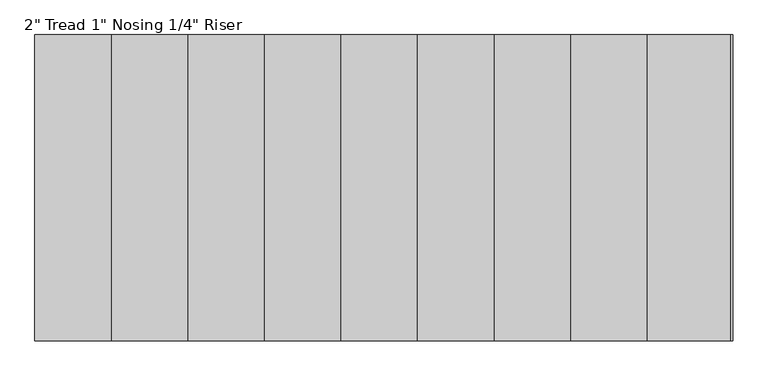
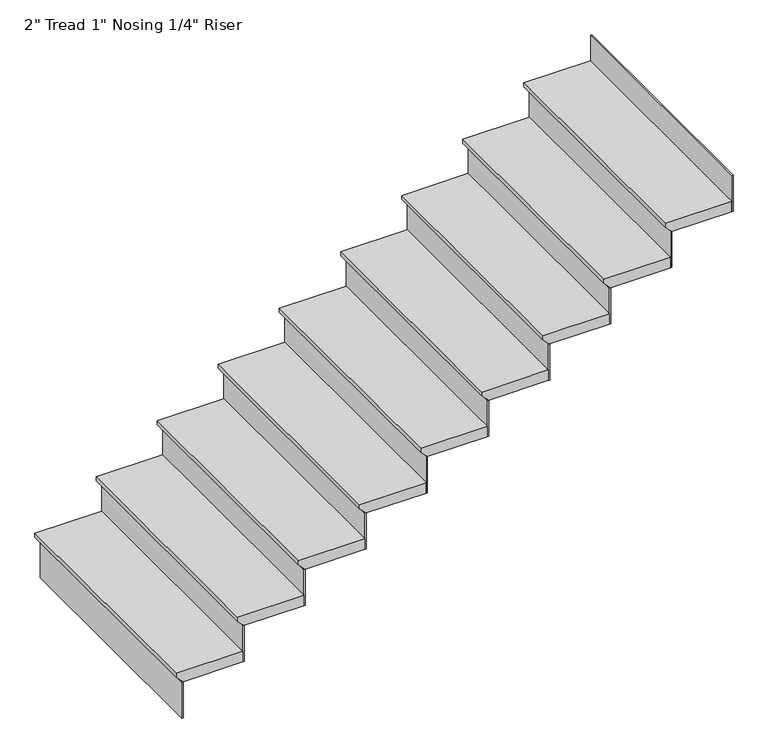
"""IFC4 building model written with IfcOpenShell, lengths in millimetres: stair flight geometry."""

import ifcopenshell
import ifcopenshell.guid

model = None  # the IFC model being written
_history = None  # IfcOwnerHistory: only IFC2X3 demands one
_inside = {}  # id of a spatial element -> (the spatial element, [elements in it])
_under = {}  # id of a project, library or spatial element -> (it, [spatial elements below it])
_declared = {}  # id of a project -> (the project, [libraries it declares])
_typed = {}  # id of a type object -> (the type object, [elements of that type])
_made_of = {}  # id of a material, layer set ... -> (it, [elements and type objects made of it])


def new_model(schema):
    """Start an empty IFC model of exactly this schema.

    Asked for "IFC4X3", IfcOpenShell would pick the latest addendum, in which some entities
    have other attributes; the version numbers below select the first issue.
    IFC2X3 requires an IfcOwnerHistory on every rooted entity: one is made here for all.
    """
    global model, _history
    if schema == "IFC4X3":
        model = ifcopenshell.file(schema_version=(4, 3, 0, 0))
    else:
        model = ifcopenshell.file(schema=schema)
    _inside.clear()
    _under.clear()
    _declared.clear()
    _typed.clear()
    _made_of.clear()
    _history = None
    if model.schema == "IFC2X3":
        org = make("IfcOrganization", Name="unknown")
        user = make(
            "IfcPersonAndOrganization",
            ThePerson=make("IfcPerson", FamilyName="unknown"),
            TheOrganization=org,
        )
        app = make(
            "IfcApplication",
            ApplicationDeveloper=org,
            Version="unknown",
            ApplicationFullName="unknown",
            ApplicationIdentifier="unknown",
        )
        _history = make(
            "IfcOwnerHistory",
            OwningUser=user,
            OwningApplication=app,
            ChangeAction="ADDED",
            CreationDate=0,
        )
    return model


def make(cls, **values):
    """One entity of the class cls with the attributes given. An attribute that is None is left unset."""
    return model.create_entity(
        cls, **{name: value for name, value in values.items() if value is not None}
    )


def rooted(cls, **values):
    """An entity with a GlobalId (a new one), such as an element, a storey or a relation."""
    return make(cls, GlobalId=ifcopenshell.guid.new(), OwnerHistory=_history, **values)


def si_unit(unit_type, name, prefix=None):
    """IfcSIUnit, for example si_unit("LENGTHUNIT", "METRE", prefix="MILLI")."""
    return make("IfcSIUnit", UnitType=unit_type, Prefix=prefix, Name=name)


def assignment(units):
    """IfcUnitAssignment: the units of a project."""
    return None if units is None else make("IfcUnitAssignment", Units=units)


def point(xyz):
    """IfcCartesianPoint."""
    return None if xyz is None else make("IfcCartesianPoint", Coordinates=xyz)


def direction(xyz):
    """IfcDirection."""
    return None if xyz is None else make("IfcDirection", DirectionRatios=xyz)


def frame(location, z_axis=None, x_axis=None):
    """IfcAxis2Placement3D, a coordinate frame: its origin and axes. An axis left out is left unset."""
    return make(
        "IfcAxis2Placement3D",
        Location=point(location),
        Axis=direction(z_axis),
        RefDirection=direction(x_axis),
    )


def origin():
    """The frame at (0, 0, 0) with its axes left unset."""
    return frame((0.0, 0.0, 0.0))


def place(relative_to, where):
    """IfcLocalPlacement: puts the frame where relative to a parent placement (None: the world)."""
    return make(
        "IfcLocalPlacement", PlacementRelTo=relative_to, RelativePlacement=where
    )


def context(
    kind, dimensions, precision=None, world=None, true_north=None, identifier=None
):
    """IfcGeometricRepresentationContext, for example the 3D "Model" context."""
    return make(
        "IfcGeometricRepresentationContext",
        ContextIdentifier=identifier,
        ContextType=kind,
        CoordinateSpaceDimension=dimensions,
        Precision=precision,
        WorldCoordinateSystem=world,
        TrueNorth=true_north,
    )


def project(units=None, contexts=None):
    """IfcProject with its units and contexts."""
    return rooted(
        "IfcProject",
        Name="project",
        RepresentationContexts=contexts,
        UnitsInContext=assignment(units),
    )


def spatial(cls, under=None, at=None, **own):
    """A site, building, storey or space (cls), placed at a placement, below another one or the project."""
    s = rooted(cls, ObjectPlacement=at, **own)
    if under is not None:
        _under.setdefault(under.id(), (under, []))[1].append(s)
    return s


def polyline(points):
    """IfcPolyline through the points."""
    return make("IfcPolyline", Points=[point(p) for p in points])


def outline(outer, holes=None, kind="AREA"):
    """IfcArbitraryClosedProfileDef: a profile drawn as a closed curve; with holes, ...WithVoids."""
    if holes is None:
        return make("IfcArbitraryClosedProfileDef", ProfileType=kind, OuterCurve=outer)
    return make(
        "IfcArbitraryProfileDefWithVoids",
        ProfileType=kind,
        OuterCurve=outer,
        InnerCurves=holes,
    )


def extrude(swept, where, along, depth):
    """IfcExtrudedAreaSolid: the profile swept, set in the frame where, extruded along a direction by depth."""
    return make(
        "IfcExtrudedAreaSolid",
        SweptArea=swept,
        Position=where,
        ExtrudedDirection=direction(along),
        Depth=depth,
    )


def shape(context_of_items, identifier, shape_type, items):
    """IfcShapeRepresentation: the items that make up one representation, for example the "Body"."""
    return make(
        "IfcShapeRepresentation",
        ContextOfItems=context_of_items,
        RepresentationIdentifier=identifier,
        RepresentationType=shape_type,
        Items=items,
    )


def source(mapping_origin, context_of_items, identifier, shape_type, items):
    """IfcRepresentationMap: a shape defined once, which mapped items show again and again."""
    return make(
        "IfcRepresentationMap",
        MappingOrigin=mapping_origin,
        MappedRepresentation=shape(context_of_items, identifier, shape_type, items),
    )


def transform(
    local_origin,
    x_axis=None,
    y_axis=None,
    z_axis=None,
    scale=None,
    scale2=None,
    scale3=None,
    uniform=True,
):
    """IfcCartesianTransformationOperator3D, or its non-uniform kind. x_axis, y_axis, z_axis: its Axis1, 2, 3."""
    if uniform:
        return make(
            "IfcCartesianTransformationOperator3D",
            Axis1=direction(x_axis),
            Axis2=direction(y_axis),
            LocalOrigin=point(local_origin),
            Scale=scale,
            Axis3=direction(z_axis),
        )
    return make(
        "IfcCartesianTransformationOperator3DnonUniform",
        Axis1=direction(x_axis),
        Axis2=direction(y_axis),
        LocalOrigin=point(local_origin),
        Scale=scale,
        Axis3=direction(z_axis),
        Scale2=scale2,
        Scale3=scale3,
    )


def mapped(mapping_source, mapping_target):
    """IfcMappedItem: shows the shape of a source again, moved by a transform."""
    return make(
        "IfcMappedItem", MappingSource=mapping_source, MappingTarget=mapping_target
    )


def made_of(thing, what):
    """Note that an element or type object is made of a material, layer set ...; save() writes the relation."""
    if what is not None:
        _made_of.setdefault(what.id(), (what, []))[1].append(thing)
    return thing


def element(
    cls,
    number,
    at=None,
    inside=None,
    cuts=None,
    type_object=None,
    material=None,
    context=None,
    identifier="Body",
    shape_type=None,
    held_by="IfcProductDefinitionShape",
    body=None,
    shapes=None,
    **own,
):
    """One element of the class cls, such as IfcWall. Its Tag is "e" and its number.

    at: its placement. inside: the storey or other place that contains it. cuts: it is an
    opening in that element (IfcRelVoidsElement). A single representation is given by context,
    identifier, shape_type and body (its items); several are given by shapes. held_by: the class
    of the entity that holds the representations. save() writes the other relations.
    """
    e = rooted(cls, Tag="e%d" % number, ObjectPlacement=at, **own)
    if body is not None:
        shapes = [shape(context, identifier, shape_type, body)]
    if shapes is not None:
        e.Representation = make(held_by, Representations=shapes)
    if inside is not None:
        _inside.setdefault(inside.id(), (inside, []))[1].append(e)
    if cuts is not None:
        rooted(
            "IfcRelVoidsElement", RelatingBuildingElement=cuts, RelatedOpeningElement=e
        )
    if type_object is not None:
        _typed.setdefault(type_object.id(), (type_object, []))[1].append(e)
    return made_of(e, material)


def aggregate(whole, parts):
    """IfcRelAggregates: a whole, such as a stair, and the parts it consists of."""
    return rooted("IfcRelAggregates", RelatingObject=whole, RelatedObjects=parts)


def save(model, path):
    """Write the relations noted so far, then the file.

    IfcRelAggregates (storeys below a building ...), IfcRelContainedInSpatialStructure (elements
    in a storey), IfcRelDefinesByType, IfcRelAssociatesMaterial and IfcRelDeclares: one each for
    every whole, place, type object, material and project.
    """
    for whole, parts in _under.values():
        aggregate(whole, parts)
    for where, things in _inside.values():
        rooted(
            "IfcRelContainedInSpatialStructure",
            RelatedElements=things,
            RelatingStructure=where,
        )
    for kind, things in _typed.values():
        rooted("IfcRelDefinesByType", RelatedObjects=things, RelatingType=kind)
    for what, things in _made_of.values():
        rooted("IfcRelAssociatesMaterial", RelatedObjects=things, RelatingMaterial=what)
    for by, libraries in _declared.values():
        rooted("IfcRelDeclares", RelatingContext=by, RelatedDefinitions=libraries)
    model.write(path)


def stair_flight_4c39f742(model_context):
    return source(origin(), model_context, "Body", "SweptSolid", [
        extrude(outline(polyline([(5747.6571429, -3197.8122732), (5747.6571429, -3502.6122732), (5728.6071429, -3502.6122732), (5703.2071429, -3477.2122732), (5696.8571429, -3477.2122732), (5696.8571429, -3197.8122732), (5747.6571429, -3197.8122732)])), frame((0.0, 8132.6265304, 0.0), z_axis=(0.0, 1.0, 0.0), x_axis=(0.0, 0.0, 1.0)), (0.0, 0.0, 1.0), 1117.6),
        extrude(outline(polyline([(-3470.8622732, 8132.6265304), (-3477.2122732, 8132.6265304), (-3477.2122732, 9250.2265304), (-3470.8622732, 9250.2265304), (-3470.8622732, 8132.6265304)])), frame((0.0, 0.0, 5522.6857143), z_axis=(0.0, 0.0, 1.0), x_axis=(1.0, 0.0, 0.0)), (0.0, 0.0, 1.0), 174.1714286),
        extrude(outline(polyline([(-3191.4622732, 8132.6265304), (-3197.8122732, 8132.6265304), (-3197.8122732, 9250.2265304), (-3191.4622732, 9250.2265304), (-3191.4622732, 8132.6265304)])), frame((0.0, 0.0, 5696.8571429), z_axis=(0.0, 0.0, 1.0), x_axis=(1.0, 0.0, 0.0)), (0.0, 0.0, 1.0), 174.1714286),
        extrude(outline(polyline([(5921.8285714, -2918.4122732), (5921.8285714, -3223.2122732), (5902.7785714, -3223.2122732), (5877.3785714, -3197.8122732), (5871.0285714, -3197.8122732), (5871.0285714, -2918.4122732), (5921.8285714, -2918.4122732)])), frame((0.0, 8132.6265304, 0.0), z_axis=(0.0, 1.0, 0.0), x_axis=(0.0, 0.0, 1.0)), (0.0, 0.0, 1.0), 1117.6),
        extrude(outline(polyline([(-2912.0622732, 8132.6265304), (-2918.4122732, 8132.6265304), (-2918.4122732, 9250.2265304), (-2912.0622732, 9250.2265304), (-2912.0622732, 8132.6265304)])), frame((0.0, 0.0, 5871.0285714), z_axis=(0.0, 0.0, 1.0), x_axis=(1.0, 0.0, 0.0)), (0.0, 0.0, 1.0), 174.1714286),
        extrude(outline(polyline([(6096.0, -2639.0122732), (6096.0, -2943.8122732), (6076.95, -2943.8122732), (6051.55, -2918.4122732), (6045.2, -2918.4122732), (6045.2, -2639.0122732), (6096.0, -2639.0122732)])), frame((0.0, 8132.6265304, 0.0), z_axis=(0.0, 1.0, 0.0), x_axis=(0.0, 0.0, 1.0)), (0.0, 0.0, 1.0), 1117.6),
        extrude(outline(polyline([(-2632.6622732, 8132.6265304), (-2639.0122732, 8132.6265304), (-2639.0122732, 9250.2265304), (-2632.6622732, 9250.2265304), (-2632.6622732, 8132.6265304)])), frame((0.0, 0.0, 6045.2), z_axis=(0.0, 0.0, 1.0), x_axis=(1.0, 0.0, 0.0)), (0.0, 0.0, 1.0), 174.1714286),
        extrude(outline(polyline([(6270.1714286, -2359.6122732), (6270.1714286, -2664.4122732), (6251.1214286, -2664.4122732), (6225.7214286, -2639.0122732), (6219.3714286, -2639.0122732), (6219.3714286, -2359.6122732), (6270.1714286, -2359.6122732)])), frame((0.0, 8132.6265304, 0.0), z_axis=(0.0, 1.0, 0.0), x_axis=(0.0, 0.0, 1.0)), (0.0, 0.0, 1.0), 1117.6),
        extrude(outline(polyline([(-2353.2622732, 8132.6265304), (-2359.6122732, 8132.6265304), (-2359.6122732, 9250.2265304), (-2353.2622732, 9250.2265304), (-2353.2622732, 8132.6265304)])), frame((0.0, 0.0, 6219.3714286), z_axis=(0.0, 0.0, 1.0), x_axis=(1.0, 0.0, 0.0)), (0.0, 0.0, 1.0), 174.1714286),
        extrude(outline(polyline([(6444.3428571, -2080.2122732), (6444.3428571, -2385.0122732), (6425.2928571, -2385.0122732), (6399.8928571, -2359.6122732), (6393.5428571, -2359.6122732), (6393.5428571, -2080.2122732), (6444.3428571, -2080.2122732)])), frame((0.0, 8132.6265304, 0.0), z_axis=(0.0, 1.0, 0.0), x_axis=(0.0, 0.0, 1.0)), (0.0, 0.0, 1.0), 1117.6),
        extrude(outline(polyline([(-2073.8622732, 8132.6265304), (-2080.2122732, 8132.6265304), (-2080.2122732, 9250.2265304), (-2073.8622732, 9250.2265304), (-2073.8622732, 8132.6265304)])), frame((0.0, 0.0, 6393.5428571), z_axis=(0.0, 0.0, 1.0), x_axis=(1.0, 0.0, 0.0)), (0.0, 0.0, 1.0), 174.1714286),
        extrude(outline(polyline([(6618.5142857, -1800.8122732), (6618.5142857, -2105.6122732), (6599.4642857, -2105.6122732), (6574.0642857, -2080.2122732), (6567.7142857, -2080.2122732), (6567.7142857, -1800.8122732), (6618.5142857, -1800.8122732)])), frame((0.0, 8132.6265304, 0.0), z_axis=(0.0, 1.0, 0.0), x_axis=(0.0, 0.0, 1.0)), (0.0, 0.0, 1.0), 1117.6),
        extrude(outline(polyline([(-1794.4622732, 8132.6265304), (-1800.8122732, 8132.6265304), (-1800.8122732, 9250.2265304), (-1794.4622732, 9250.2265304), (-1794.4622732, 8132.6265304)])), frame((0.0, 0.0, 6567.7142857), z_axis=(0.0, 0.0, 1.0), x_axis=(1.0, 0.0, 0.0)), (0.0, 0.0, 1.0), 174.1714286),
        extrude(outline(polyline([(6792.6857143, -1521.4122732), (6792.6857143, -1826.2122732), (6773.6357143, -1826.2122732), (6748.2357143, -1800.8122732), (6741.8857143, -1800.8122732), (6741.8857143, -1521.4122732), (6792.6857143, -1521.4122732)])), frame((0.0, 8132.6265304, 0.0), z_axis=(0.0, 1.0, 0.0), x_axis=(0.0, 0.0, 1.0)), (0.0, 0.0, 1.0), 1117.6),
        extrude(outline(polyline([(-1515.0622732, 8132.6265304), (-1521.4122732, 8132.6265304), (-1521.4122732, 9250.2265304), (-1515.0622732, 9250.2265304), (-1515.0622732, 8132.6265304)])), frame((0.0, 0.0, 6741.8857143), z_axis=(0.0, 0.0, 1.0), x_axis=(1.0, 0.0, 0.0)), (0.0, 0.0, 1.0), 174.1714286),
        extrude(outline(polyline([(6966.8571429, -1242.0122732), (6966.8571429, -1546.8122732), (6947.8071429, -1546.8122732), (6922.4071429, -1521.4122732), (6916.0571429, -1521.4122732), (6916.0571429, -1242.0122732), (6966.8571429, -1242.0122732)])), frame((0.0, 8132.6265304, 0.0), z_axis=(0.0, 1.0, 0.0), x_axis=(0.0, 0.0, 1.0)), (0.0, 0.0, 1.0), 1117.6),
        extrude(outline(polyline([(-1235.6622732, 8132.6265304), (-1242.0122732, 8132.6265304), (-1242.0122732, 9250.2265304), (-1235.6622732, 9250.2265304), (-1235.6622732, 8132.6265304)])), frame((0.0, 0.0, 6916.0571429), z_axis=(0.0, 0.0, 1.0), x_axis=(1.0, 0.0, 0.0)), (0.0, 0.0, 1.0), 174.1714286),
        extrude(outline(polyline([(-956.2622732, 8132.6265304), (-962.6122732, 8132.6265304), (-962.6122732, 9250.2265304), (-956.2622732, 9250.2265304), (-956.2622732, 8132.6265304)])), frame((0.0, 0.0, 7090.2285714), z_axis=(0.0, 0.0, 1.0), x_axis=(1.0, 0.0, 0.0)), (0.0, 0.0, 1.0), 174.1714286),
        extrude(outline(polyline([(7141.0285714, -962.6122732), (7141.0285714, -1267.4122732), (7121.9785714, -1267.4122732), (7096.5785714, -1242.0122732), (7090.2285714, -1242.0122732), (7090.2285714, -962.6122732), (7141.0285714, -962.6122732)])), frame((0.0, 8132.6265304, 0.0), z_axis=(0.0, 1.0, 0.0), x_axis=(0.0, 0.0, 1.0)), (0.0, 0.0, 1.0), 1117.6),
    ])


if __name__ == "__main__":
    model = new_model("IFC4")
    model_context = context("Model", 3, world=origin())
    ifc_project = project(units=[si_unit("LENGTHUNIT", "METRE", prefix="MILLI")], contexts=[model_context])
    site = spatial("IfcSite", under=ifc_project)
    building = spatial("IfcBuilding", under=site)
    placement = place(None, origin())
    stair_flight_shape = stair_flight_4c39f742(model_context)
    element("IfcStairFlight", 1, ObjectType="2\" Tread 1\" Nosing 1/4\" Riser", at=placement, inside=building, context=model_context, shape_type="MappedRepresentation", body=[
        mapped(stair_flight_shape, transform((0.0, 0.0, 0.0), x_axis=(1.0, 0.0, 0.0), y_axis=(0.0, 1.0, 0.0), z_axis=(0.0, 0.0, 1.0))),
    ])
    save(model, "model.ifc")
